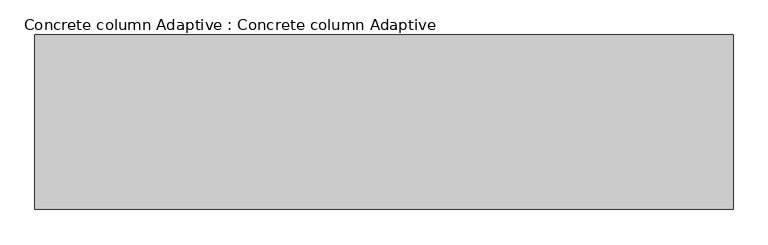
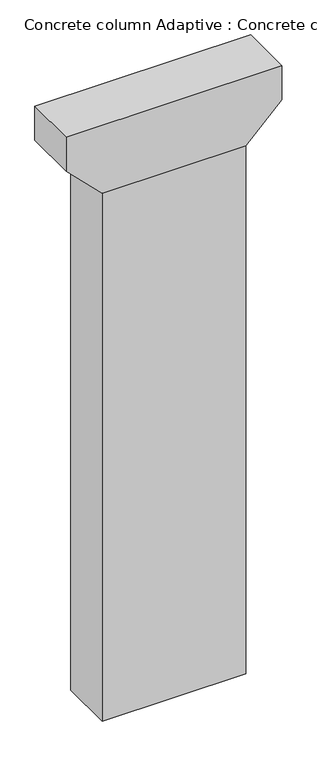
"""IFC4 building model written with IfcOpenShell, lengths in millimetres: proxy geometry, Concrete column Adaptive : Concrete column Adaptive."""

import ifcopenshell
import ifcopenshell.guid

model = None  # the IFC model being written
_history = None  # IfcOwnerHistory: only IFC2X3 demands one
_inside = {}  # id of a spatial element -> (the spatial element, [elements in it])
_under = {}  # id of a project, library or spatial element -> (it, [spatial elements below it])
_declared = {}  # id of a project -> (the project, [libraries it declares])
_typed = {}  # id of a type object -> (the type object, [elements of that type])
_made_of = {}  # id of a material, layer set ... -> (it, [elements and type objects made of it])


def new_model(schema):
    """Start an empty IFC model of exactly this schema.

    Asked for "IFC4X3", IfcOpenShell would pick the latest addendum, in which some entities
    have other attributes; the version numbers below select the first issue.
    IFC2X3 requires an IfcOwnerHistory on every rooted entity: one is made here for all.
    """
    global model, _history
    if schema == "IFC4X3":
        model = ifcopenshell.file(schema_version=(4, 3, 0, 0))
    else:
        model = ifcopenshell.file(schema=schema)
    _inside.clear()
    _under.clear()
    _declared.clear()
    _typed.clear()
    _made_of.clear()
    _history = None
    if model.schema == "IFC2X3":
        org = make("IfcOrganization", Name="unknown")
        user = make(
            "IfcPersonAndOrganization",
            ThePerson=make("IfcPerson", FamilyName="unknown"),
            TheOrganization=org,
        )
        app = make(
            "IfcApplication",
            ApplicationDeveloper=org,
            Version="unknown",
            ApplicationFullName="unknown",
            ApplicationIdentifier="unknown",
        )
        _history = make(
            "IfcOwnerHistory",
            OwningUser=user,
            OwningApplication=app,
            ChangeAction="ADDED",
            CreationDate=0,
        )
    return model


def make(cls, **values):
    """One entity of the class cls with the attributes given. An attribute that is None is left unset."""
    return model.create_entity(
        cls, **{name: value for name, value in values.items() if value is not None}
    )


def rooted(cls, **values):
    """An entity with a GlobalId (a new one), such as an element, a storey or a relation."""
    return make(cls, GlobalId=ifcopenshell.guid.new(), OwnerHistory=_history, **values)


def si_unit(unit_type, name, prefix=None):
    """IfcSIUnit, for example si_unit("LENGTHUNIT", "METRE", prefix="MILLI")."""
    return make("IfcSIUnit", UnitType=unit_type, Prefix=prefix, Name=name)


def assignment(units):
    """IfcUnitAssignment: the units of a project."""
    return None if units is None else make("IfcUnitAssignment", Units=units)


def point(xyz):
    """IfcCartesianPoint."""
    return None if xyz is None else make("IfcCartesianPoint", Coordinates=xyz)


def direction(xyz):
    """IfcDirection."""
    return None if xyz is None else make("IfcDirection", DirectionRatios=xyz)


def frame(location, z_axis=None, x_axis=None):
    """IfcAxis2Placement3D, a coordinate frame: its origin and axes. An axis left out is left unset."""
    return make(
        "IfcAxis2Placement3D",
        Location=point(location),
        Axis=direction(z_axis),
        RefDirection=direction(x_axis),
    )


def origin():
    """The frame at (0, 0, 0) with its axes left unset."""
    return frame((0.0, 0.0, 0.0))


def origin_with_axes():
    """The frame at (0, 0, 0) with the z axis (0, 0, 1) and the x axis (1, 0, 0) written out."""
    return frame((0.0, 0.0, 0.0), z_axis=(0.0, 0.0, 1.0), x_axis=(1.0, 0.0, 0.0))


def place(relative_to, where):
    """IfcLocalPlacement: puts the frame where relative to a parent placement (None: the world)."""
    return make(
        "IfcLocalPlacement", PlacementRelTo=relative_to, RelativePlacement=where
    )


def context(
    kind, dimensions, precision=None, world=None, true_north=None, identifier=None
):
    """IfcGeometricRepresentationContext, for example the 3D "Model" context."""
    return make(
        "IfcGeometricRepresentationContext",
        ContextIdentifier=identifier,
        ContextType=kind,
        CoordinateSpaceDimension=dimensions,
        Precision=precision,
        WorldCoordinateSystem=world,
        TrueNorth=true_north,
    )


def project(units=None, contexts=None):
    """IfcProject with its units and contexts."""
    return rooted(
        "IfcProject",
        Name="project",
        RepresentationContexts=contexts,
        UnitsInContext=assignment(units),
    )


def spatial(cls, under=None, at=None, **own):
    """A site, building, storey or space (cls), placed at a placement, below another one or the project."""
    s = rooted(cls, ObjectPlacement=at, **own)
    if under is not None:
        _under.setdefault(under.id(), (under, []))[1].append(s)
    return s


def polyline(points):
    """IfcPolyline through the points."""
    return make("IfcPolyline", Points=[point(p) for p in points])


def outline(outer, holes=None, kind="AREA"):
    """IfcArbitraryClosedProfileDef: a profile drawn as a closed curve; with holes, ...WithVoids."""
    if holes is None:
        return make("IfcArbitraryClosedProfileDef", ProfileType=kind, OuterCurve=outer)
    return make(
        "IfcArbitraryProfileDefWithVoids",
        ProfileType=kind,
        OuterCurve=outer,
        InnerCurves=holes,
    )


def extrude(swept, where, along, depth):
    """IfcExtrudedAreaSolid: the profile swept, set in the frame where, extruded along a direction by depth."""
    return make(
        "IfcExtrudedAreaSolid",
        SweptArea=swept,
        Position=where,
        ExtrudedDirection=direction(along),
        Depth=depth,
    )


def shape(context_of_items, identifier, shape_type, items):
    """IfcShapeRepresentation: the items that make up one representation, for example the "Body"."""
    return make(
        "IfcShapeRepresentation",
        ContextOfItems=context_of_items,
        RepresentationIdentifier=identifier,
        RepresentationType=shape_type,
        Items=items,
    )


def source(mapping_origin, context_of_items, identifier, shape_type, items):
    """IfcRepresentationMap: a shape defined once, which mapped items show again and again."""
    return make(
        "IfcRepresentationMap",
        MappingOrigin=mapping_origin,
        MappedRepresentation=shape(context_of_items, identifier, shape_type, items),
    )


def transform(
    local_origin,
    x_axis=None,
    y_axis=None,
    z_axis=None,
    scale=None,
    scale2=None,
    scale3=None,
    uniform=True,
):
    """IfcCartesianTransformationOperator3D, or its non-uniform kind. x_axis, y_axis, z_axis: its Axis1, 2, 3."""
    if uniform:
        return make(
            "IfcCartesianTransformationOperator3D",
            Axis1=direction(x_axis),
            Axis2=direction(y_axis),
            LocalOrigin=point(local_origin),
            Scale=scale,
            Axis3=direction(z_axis),
        )
    return make(
        "IfcCartesianTransformationOperator3DnonUniform",
        Axis1=direction(x_axis),
        Axis2=direction(y_axis),
        LocalOrigin=point(local_origin),
        Scale=scale,
        Axis3=direction(z_axis),
        Scale2=scale2,
        Scale3=scale3,
    )


def mapped(mapping_source, mapping_target):
    """IfcMappedItem: shows the shape of a source again, moved by a transform."""
    return make(
        "IfcMappedItem", MappingSource=mapping_source, MappingTarget=mapping_target
    )


def made_of(thing, what):
    """Note that an element or type object is made of a material, layer set ...; save() writes the relation."""
    if what is not None:
        _made_of.setdefault(what.id(), (what, []))[1].append(thing)
    return thing


def element(
    cls,
    number,
    at=None,
    inside=None,
    cuts=None,
    type_object=None,
    material=None,
    context=None,
    identifier="Body",
    shape_type=None,
    held_by="IfcProductDefinitionShape",
    body=None,
    shapes=None,
    **own,
):
    """One element of the class cls, such as IfcWall. Its Tag is "e" and its number.

    at: its placement. inside: the storey or other place that contains it. cuts: it is an
    opening in that element (IfcRelVoidsElement). A single representation is given by context,
    identifier, shape_type and body (its items); several are given by shapes. held_by: the class
    of the entity that holds the representations. save() writes the other relations.
    """
    e = rooted(cls, Tag="e%d" % number, ObjectPlacement=at, **own)
    if body is not None:
        shapes = [shape(context, identifier, shape_type, body)]
    if shapes is not None:
        e.Representation = make(held_by, Representations=shapes)
    if inside is not None:
        _inside.setdefault(inside.id(), (inside, []))[1].append(e)
    if cuts is not None:
        rooted(
            "IfcRelVoidsElement", RelatingBuildingElement=cuts, RelatedOpeningElement=e
        )
    if type_object is not None:
        _typed.setdefault(type_object.id(), (type_object, []))[1].append(e)
    return made_of(e, material)


def aggregate(whole, parts):
    """IfcRelAggregates: a whole, such as a stair, and the parts it consists of."""
    return rooted("IfcRelAggregates", RelatingObject=whole, RelatedObjects=parts)


def save(model, path):
    """Write the relations noted so far, then the file.

    IfcRelAggregates (storeys below a building ...), IfcRelContainedInSpatialStructure (elements
    in a storey), IfcRelDefinesByType, IfcRelAssociatesMaterial and IfcRelDeclares: one each for
    every whole, place, type object, material and project.
    """
    for whole, parts in _under.values():
        aggregate(whole, parts)
    for where, things in _inside.values():
        rooted(
            "IfcRelContainedInSpatialStructure",
            RelatedElements=things,
            RelatingStructure=where,
        )
    for kind, things in _typed.values():
        rooted("IfcRelDefinesByType", RelatedObjects=things, RelatingType=kind)
    for what, things in _made_of.values():
        rooted("IfcRelAssociatesMaterial", RelatedObjects=things, RelatingMaterial=what)
    for by, libraries in _declared.values():
        rooted("IfcRelDeclares", RelatingContext=by, RelatedDefinitions=libraries)
    model.write(path)


def concrete_column_adaptive_concrete_column_adaptive_b0f9f52a(model_context):
    return source(origin(), model_context, "Body", "SweptSolid", [
        extrude(outline(polyline([(35017.0, 6000.0), (35017.0, -6000.0), (33017.0, -6000.0), (31017.0, -4000.0), (31017.0, 4000.0), (33017.0, 6000.0), (35017.0, 6000.0)])), frame((0.0, -1500.0, 0.0), z_axis=(0.0, 1.0, 0.0), x_axis=(0.0, 0.0, 1.0)), (0.0, 0.0, 1.0), 3000.0),
        extrude(outline(polyline([(-4000.0, -1500.0), (-4000.0, 1500.0), (4000.0, 1500.0), (4000.0, -1500.0), (-4000.0, -1500.0)])), origin_with_axes(), (0.0, 0.0, 1.0), 31017.0),
    ])


if __name__ == "__main__":
    model = new_model("IFC4")
    model_context = context("Model", 3, world=origin())
    ifc_project = project(units=[si_unit("LENGTHUNIT", "METRE", prefix="MILLI")], contexts=[model_context])
    site = spatial("IfcSite", under=ifc_project)
    building = spatial("IfcBuilding", under=site)
    placement = place(None, origin())
    concrete_column_adaptive_concrete_column_adaptive_shape = concrete_column_adaptive_concrete_column_adaptive_b0f9f52a(model_context)
    element("IfcBuildingElementProxy", 1, Name="Concrete column Adaptive : Concrete column Adaptive", ObjectType="Concrete column Adaptive : Concrete column Adaptive", at=placement, inside=building, context=model_context, shape_type="MappedRepresentation", body=[
        mapped(concrete_column_adaptive_concrete_column_adaptive_shape, transform((0.0, 0.0, 0.0), x_axis=(1.0, 0.0, 0.0), y_axis=(0.0, 1.0, 0.0), z_axis=(0.0, 0.0, 1.0))),
    ])
    save(model, "model.ifc")

# Revit data of these elements
# Type "Concrete column Adaptive : Concrete column Adaptive"
#   Height [instance default] = 30000 mm
#   Default Elevation = 0
# Element 1 (IfcBuildingElementProxy, "Concrete column Adaptive : Concrete column Adaptive")
#   Height = 31017 mm
#   Materials on its faces: "Default Wall"
# Materials
#   "Default Wall": class "Miscellaneous", colour RGB 128 128 128, transparency 0, Comments = "Rendering appearance not upgraded Rendering appearance not upgraded ", Cost = 0
